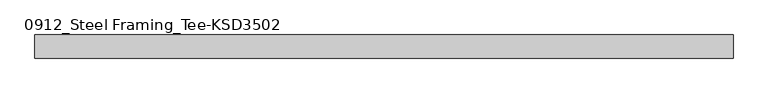
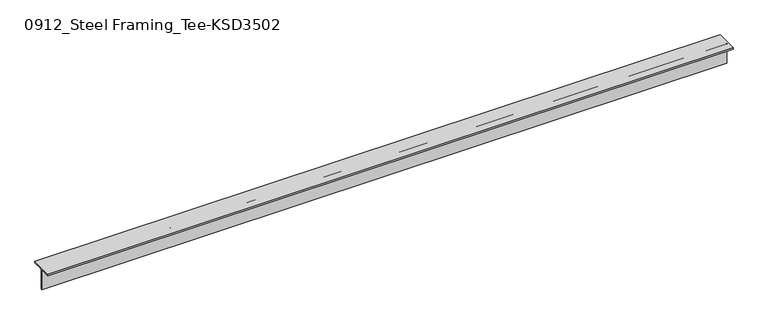
"""IFC4 building model written with IfcOpenShell, lengths in millimetres: member geometry, 0912_Steel Framing_Tee-KSD3502 : H_SB_ASB_CT-150x150x6.5x9."""

from ifc_helpers import new_model, si_unit, point, frame, frame_2d, origin, place, context, project, spatial, polyline, circle_curve, trimmed, segment, composite_curve, outline, extrude, source, transform, mapped, element, save


def member_0912_steel_framing_tee_ksd3502_a5ad979a(model_context):
    return source(origin(), model_context, "Body", "SweptSolid", [
        extrude(outline(composite_curve([segment(polyline([(-75.0, 75.0), (75.0, 75.0), (75.0, 66.0), (16.25, 66.0)]), True, "CONTINUOUS"), segment(trimmed(circle_curve(frame_2d((16.25, 53.0)), 13.0), [point((16.25, 66.0))], [point((3.25, 53.0))], True, "CARTESIAN"), True, "CONTINUOUS"), segment(polyline([(3.25, 53.0), (3.25, -75.0), (-3.25, -75.0), (-3.25, 53.0)]), True, "CONTINUOUS"), segment(trimmed(circle_curve(frame_2d((-16.25, 53.0)), 13.0), [point((-3.25, 53.0))], [point((-16.25, 66.0))], True, "CARTESIAN"), True, "CONTINUOUS"), segment(polyline([(-16.25, 66.0), (-75.0, 66.0), (-75.0, 75.0)]), True, "CONTINUOUS")], self_intersect=False)), frame((-2227.6, 0.0, 0.0), z_axis=(1.0, 0.0, 0.0), x_axis=(0.0, 1.0, 0.0)), (0.0, 0.0, 1.0), 4533.0),
    ])


if __name__ == "__main__":
    model = new_model("IFC4")
    model_context = context("Model", 3, world=origin())
    ifc_project = project(units=[si_unit("LENGTHUNIT", "METRE", prefix="MILLI")], contexts=[model_context])
    site = spatial("IfcSite", under=ifc_project)
    building = spatial("IfcBuilding", under=site)
    placement = place(None, origin())
    member_0912_steel_framing_tee_ksd3502_shape = member_0912_steel_framing_tee_ksd3502_a5ad979a(model_context)
    element("IfcMember", 1, ObjectType="0912_Steel Framing_Tee-KSD3502 : H_SB_ASB_CT-150x150x6.5x9", at=placement, inside=building, context=model_context, shape_type="MappedRepresentation", body=[
        mapped(member_0912_steel_framing_tee_ksd3502_shape, transform((0.0, 0.0, 0.0), x_axis=(1.0, 0.0, 0.0), y_axis=(0.0, 1.0, 0.0), z_axis=(0.0, 0.0, 1.0))),
    ])
    save(model, "model.ifc")

# Revit data of these elements
# Type "0912_Steel Framing_Tee-KSD3502 : H_SB_ASB_CT-150x150x6.5x9"
#   H_WM Code_1 = "S01AA003-00001 | Main Steel Structure Fabrication Work | Shelter/Building | Light Steel - Standard (30KG/M>Weight) | Material: (   )"
#   H_WM Code_2 = "S03AA029-00001 | Main Steel Structure Erection Work | Shelter/Building | Light Steel (30KG/M>Weight) | Material: (   )"
#   H_WM Code_3 = "S01AA010-00001 | Main Steel Structure Fabrication Work | Shelter/Building | Steel Painting/Coating | for Non-Fireproofed Steel Surface, Surface Preparation, Primer, Second & Final Coat | Material: (   )"
#   H_Q'ty Cal Type Tag = "SB-Q2"
#   Width = 15.0 cm
#   Web Thickness = 0.65 cm
#   Web Fillet = 1.3 cm
#   Section Area = 23.39 cm²
#   Perimeter = 0.60 m²/m
#   Nominal Weight = 18.40 kgf/m
#   Height = 15.0 cm
#   Flange Thickness = 0.9 cm
#   Centroid Vertical = 7.5 cm
#   Centroid Horizontal = 7.5 cm
#   Length [instance default] = 1.5000 m
#   Structural Material [instance default] = Steel, 45-345
#   Warping Constant = (empty or 0)
#   Torsional Moment of Inertia = 0
#   Section Name Key = ""
#   Plastic Modulus weak axis = 0
#   Plastic Modulus strong axis = 0
#   Moment of Inertia weak axis = 0
#   Moment of Inertia strong axis = 0
#   Elastic Modulus weak axis = 0
#   Elastic Modulus strong axis = 0
#   Bolt Spacing = 0
#   Assembly Code = ""
# Element 1 (IfcMember, "0912_Steel Framing_Tee-KSD3502 : H_SB_ASB_CT-150x150x6.5x9")
#   Structural Material = none
# Materials
#   "Steel, 45-345": class "Metal", colour RGB 189 187 185, transparency 0, Description = "Steel 345 MPa", Cost = 0
